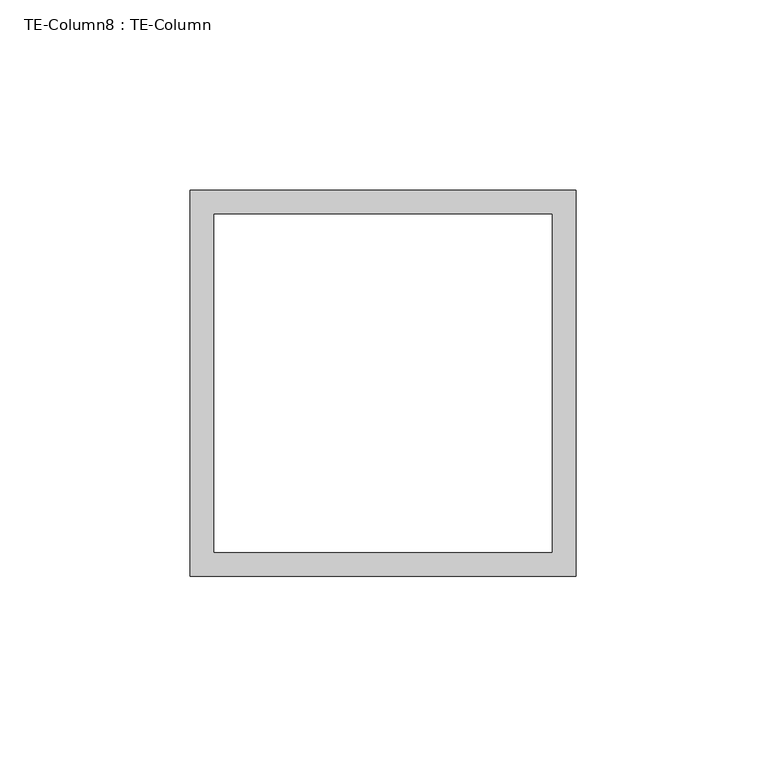
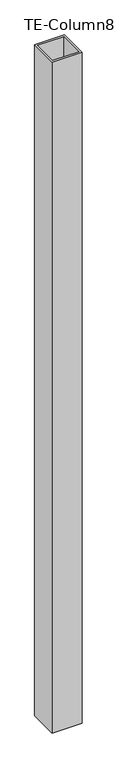
"""IFC4 building model written with IfcOpenShell, lengths in millimetres: proxy geometry, TE-Column8 : TE-Column."""

from ifc_helpers import new_model, si_unit, frame, origin, place, context, project, spatial, polyline, outline, extrude, source, transform, mapped, element, save


def te_column8_te_column_a4862150(model_context):
    return source(origin(), model_context, "Body", "SweptSolid", [
        extrude(outline(polyline([(587365.8934739, -536315.9913841), (587467.4934739, -536315.9913841), (587467.4934739, -536417.5913841), (587365.8934739, -536417.5913841), (587365.8934739, -536315.9913841)]), holes=[polyline([(587372.2434739, -536411.2413841), (587461.1434739, -536411.2413841), (587461.1434739, -536322.3413841), (587372.2434739, -536322.3413841), (587372.2434739, -536411.2413841)])]), frame((0.0, 0.0, 28.575), z_axis=(0.0, 0.0, 1.0), x_axis=(1.0, 0.0, 0.0)), (0.0, 0.0, 1.0), 2406.65),
    ])


if __name__ == "__main__":
    model = new_model("IFC4")
    model_context = context("Model", 3, world=origin())
    ifc_project = project(units=[si_unit("LENGTHUNIT", "METRE", prefix="MILLI")], contexts=[model_context])
    site = spatial("IfcSite", under=ifc_project)
    building = spatial("IfcBuilding", under=site)
    placement = place(None, origin())
    te_column8_te_column_shape = te_column8_te_column_a4862150(model_context)
    element("IfcBuildingElementProxy", 1, Name="TE-Column8 : TE-Column", ObjectType="TE-Column8 : TE-Column", at=placement, inside=building, context=model_context, shape_type="MappedRepresentation", body=[
        mapped(te_column8_te_column_shape, transform((0.0, 0.0, 0.0), x_axis=(1.0, 0.0, 0.0), y_axis=(0.0, 1.0, 0.0), z_axis=(0.0, 0.0, 1.0))),
    ])
    save(model, "model.ifc")

# Revit data of these elements
# Element 1 (IfcBuildingElementProxy, "TE-Column8 : TE-Column")
#   Materials on its faces: "4\"X4\" GALV. HSS TUBING"
# Materials
#   "4\"X4\" GALV. HSS TUBING": class "Generic", colour RGB 211 211 207, transparency 0, Cost = 0
